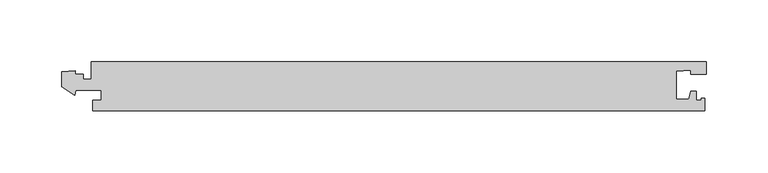
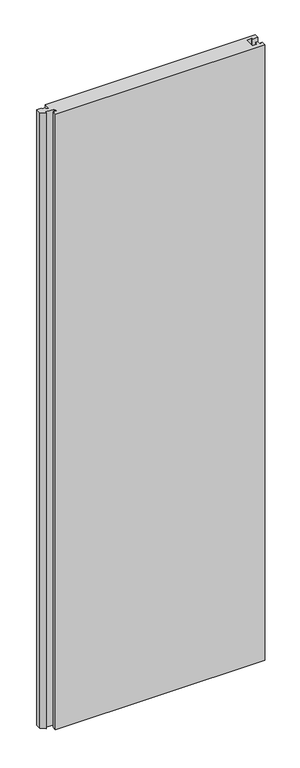
"""IFC4 building model written with IfcOpenShell, lengths in millimetres: proxy geometry, Generic Models 5:Generic Models 5:321804:Generic Models 5:321804 : Generic Models 5:Generic Models 5:321804:6 : Generic Models 5:Generic Models 5:321804:Generic Models 5:321804 : Generic Models 5:Generic Models 5:321804:300761."""

from ifc_helpers import new_model, si_unit, frame, origin, place, context, project, spatial, polyline, outline, extrude, source, transform, mapped, element, save


def generic_models_1d8c0450(model_context):
    return source(origin(), model_context, "Body", "SweptSolid", [
        extrude(outline(polyline([(593294.8386129, -536499.5289881), (593296.5802827, -536493.0289881), (593301.0302827, -536493.0289881), (593301.0302827, -536500.5289881), (593304.9802827, -536500.5289881), (593304.9802827, -536499.0289881), (593307.9802827, -536499.0289881), (593307.9802827, -536509.0289881), (592810.4802827, -536509.0289881), (592810.4802827, -536500.5289881), (592817.4302827, -536500.5289881), (592817.4302827, -536492.5289881), (592796.7142572, -536492.5289881), (592795.6617846, -536496.4568695), (592784.9802827, -536489.3495044), (592784.9802827, -536477.4913634), (592795.9802827, -536476.5289881), (592795.9802827, -536479.2289881), (592802.6052827, -536479.2289881), (592802.6052827, -536483.5289881), (592809.2302827, -536483.5289881), (592809.2302827, -536469.0289881), (593309.2302827, -536469.0289881), (593309.2302827, -536479.2289881), (593296.4802827, -536479.2289881), (593296.4802827, -536475.9833338), (593284.4802827, -536477.0331978), (593284.4802827, -536499.5289881), (593294.8386129, -536499.5289881)])), frame((0.0, 0.0, 8541.4301003), z_axis=(0.0, 0.0, 1.0), x_axis=(1.0, 0.0, 0.0)), (0.0, 0.0, 1.0), 1547.5394805),
    ])


if __name__ == "__main__":
    model = new_model("IFC4")
    model_context = context("Model", 3, world=origin())
    ifc_project = project(units=[si_unit("LENGTHUNIT", "METRE", prefix="MILLI")], contexts=[model_context])
    site = spatial("IfcSite", under=ifc_project)
    building = spatial("IfcBuilding", under=site)
    placement = place(None, origin())
    generic_models_shape = generic_models_1d8c0450(model_context)
    element("IfcBuildingElementProxy", 1, Name="Generic Models 5:Generic Models 5:321804:Generic Models 5:321804 : Generic Models 5:Generic Models 5:321804:6 : Generic Models 5:Generic Models 5:321804:Generic Models 5:321804 : Generic Models 5:Generic Models 5:321804:300761", ObjectType="Generic Models 5:Generic Models 5:321804:Generic Models 5:321804 : Generic Models 5:Generic Models 5:321804:6 : Generic Models 5:Generic Models 5:321804:Generic Models 5:321804 : Generic Models 5:Generic Models 5:321804:300761", at=placement, inside=building, context=model_context, shape_type="MappedRepresentation", body=[
        mapped(generic_models_shape, transform((0.0, 0.0, 0.0), x_axis=(1.0, 0.0, 0.0), y_axis=(0.0, 1.0, 0.0), z_axis=(0.0, 0.0, 1.0))),
    ])
    save(model, "model.ifc")

# Revit data of these elements
# Type "Generic Models 5:Generic Models 5:321804:Generic Models 5:321804 : Generic Models 5:Generic Models 5:321804:6 : Generic Models 5:Generic Models 5:321804:Generic Models 5:321804 : Generic Models 5:Generic Models 5:321804:300761"
#   NameOverride = "Generic Models 5:Generic Models 5:321804:Generic Models 5:321804 : Generic Models 5:Generic Models 5:321804:300761"
#   ObjectTypeOverride = "Generic Models 5:321804 : Generic Models 5:Generic Models 5:321804"
#   Reference = "Generic Models 5"
#   Tag = "300761"
# Element 1 (IfcBuildingElementProxy, "Generic Models 5:Generic Models 5:321804:Generic Models 5:321804 : Generic Models 5:Generic Models 5:321804:6 : Generic Models 5:Generic Models 5:321804:Generic Models 5:321804 : Generic Models 5:Generic Models 5:321804:300761")
#   Materials on its faces: "POLYCARBONATE PANEL - ARCOPLUS 547"
# Materials
#   "POLYCARBONATE PANEL - ARCOPLUS 547": class "Unassigned", colour RGB 202 225 249, transparency 0.45, Cost = 0
